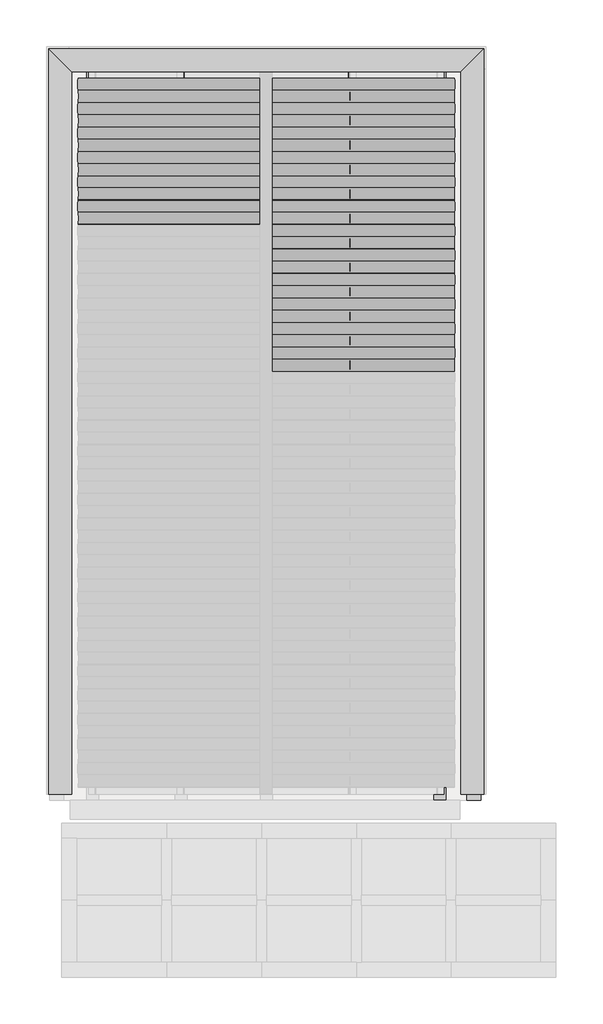
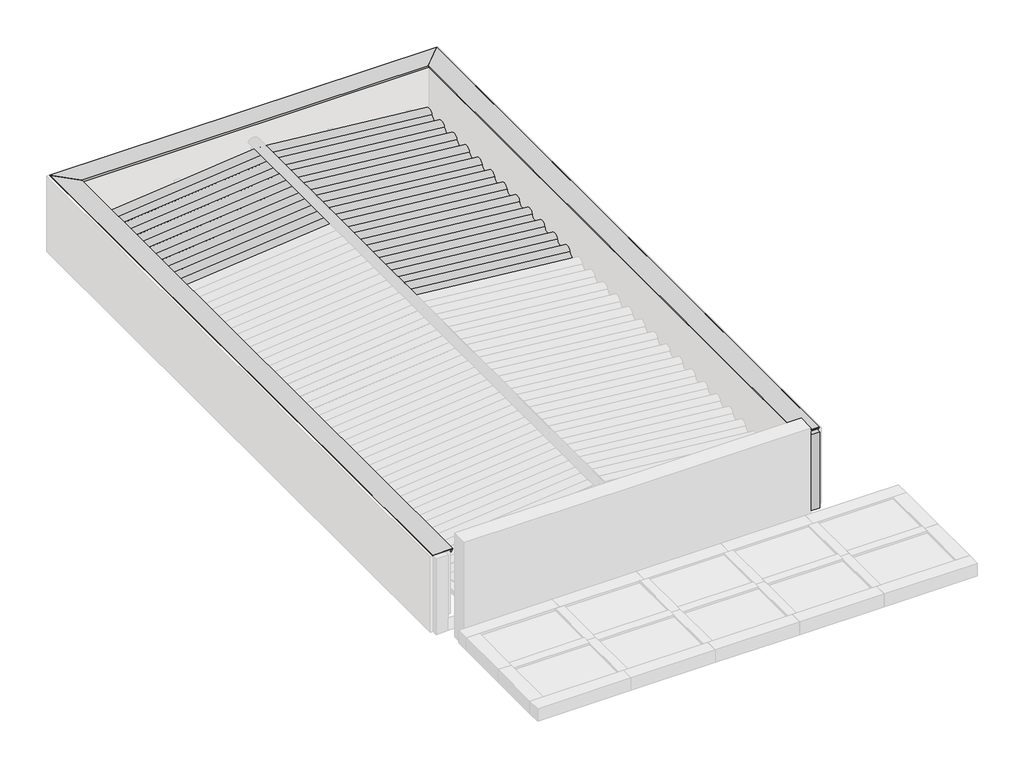
# One storey, part 3 of 3: 32 beams, 11 columns, 2 proxies.
"""IFC4 building model written with IfcOpenShell, lengths in millimetres."""

import ifcopenshell
import ifcopenshell.guid

model = None  # the IFC model being written
_history = None  # IfcOwnerHistory: only IFC2X3 demands one
_inside = {}  # id of a spatial element -> (the spatial element, [elements in it])
_under = {}  # id of a project, library or spatial element -> (it, [spatial elements below it])
_declared = {}  # id of a project -> (the project, [libraries it declares])
_typed = {}  # id of a type object -> (the type object, [elements of that type])
_made_of = {}  # id of a material, layer set ... -> (it, [elements and type objects made of it])


def new_model(schema):
    """Start an empty IFC model of exactly this schema.

    Asked for "IFC4X3", IfcOpenShell would pick the latest addendum, in which some entities
    have other attributes; the version numbers below select the first issue.
    IFC2X3 requires an IfcOwnerHistory on every rooted entity: one is made here for all.
    """
    global model, _history
    if schema == "IFC4X3":
        model = ifcopenshell.file(schema_version=(4, 3, 0, 0))
    else:
        model = ifcopenshell.file(schema=schema)
    _inside.clear()
    _under.clear()
    _declared.clear()
    _typed.clear()
    _made_of.clear()
    _history = None
    if model.schema == "IFC2X3":
        org = make("IfcOrganization", Name="unknown")
        user = make(
            "IfcPersonAndOrganization",
            ThePerson=make("IfcPerson", FamilyName="unknown"),
            TheOrganization=org,
        )
        app = make(
            "IfcApplication",
            ApplicationDeveloper=org,
            Version="unknown",
            ApplicationFullName="unknown",
            ApplicationIdentifier="unknown",
        )
        _history = make(
            "IfcOwnerHistory",
            OwningUser=user,
            OwningApplication=app,
            ChangeAction="ADDED",
            CreationDate=0,
        )
    return model


def make(cls, **values):
    """One entity of the class cls with the attributes given. An attribute that is None is left unset."""
    return model.create_entity(
        cls, **{name: value for name, value in values.items() if value is not None}
    )


def rooted(cls, **values):
    """An entity with a GlobalId (a new one), such as an element, a storey or a relation."""
    return make(cls, GlobalId=ifcopenshell.guid.new(), OwnerHistory=_history, **values)


def si_unit(unit_type, name, prefix=None):
    """IfcSIUnit, for example si_unit("LENGTHUNIT", "METRE", prefix="MILLI")."""
    return make("IfcSIUnit", UnitType=unit_type, Prefix=prefix, Name=name)


def assignment(units):
    """IfcUnitAssignment: the units of a project."""
    return None if units is None else make("IfcUnitAssignment", Units=units)


def point(xyz):
    """IfcCartesianPoint."""
    return None if xyz is None else make("IfcCartesianPoint", Coordinates=xyz)


def direction(xyz):
    """IfcDirection."""
    return None if xyz is None else make("IfcDirection", DirectionRatios=xyz)


def frame(location, z_axis=None, x_axis=None):
    """IfcAxis2Placement3D, a coordinate frame: its origin and axes. An axis left out is left unset."""
    return make(
        "IfcAxis2Placement3D",
        Location=point(location),
        Axis=direction(z_axis),
        RefDirection=direction(x_axis),
    )


def frame_2d(location, x_axis=None):
    """IfcAxis2Placement2D, a coordinate frame in the plane: its origin and x axis."""
    return make(
        "IfcAxis2Placement2D", Location=point(location), RefDirection=direction(x_axis)
    )


def origin():
    """The frame at (0, 0, 0) with its axes left unset."""
    return frame((0.0, 0.0, 0.0))


def place(relative_to, where):
    """IfcLocalPlacement: puts the frame where relative to a parent placement (None: the world)."""
    return make(
        "IfcLocalPlacement", PlacementRelTo=relative_to, RelativePlacement=where
    )


def context(
    kind, dimensions, precision=None, world=None, true_north=None, identifier=None
):
    """IfcGeometricRepresentationContext, for example the 3D "Model" context."""
    return make(
        "IfcGeometricRepresentationContext",
        ContextIdentifier=identifier,
        ContextType=kind,
        CoordinateSpaceDimension=dimensions,
        Precision=precision,
        WorldCoordinateSystem=world,
        TrueNorth=true_north,
    )


def project(units=None, contexts=None):
    """IfcProject with its units and contexts."""
    return rooted(
        "IfcProject",
        Name="project",
        RepresentationContexts=contexts,
        UnitsInContext=assignment(units),
    )


def spatial(cls, under=None, at=None, **own):
    """A site, building, storey or space (cls), placed at a placement, below another one or the project."""
    s = rooted(cls, ObjectPlacement=at, **own)
    if under is not None:
        _under.setdefault(under.id(), (under, []))[1].append(s)
    return s


def polyline(points):
    """IfcPolyline through the points."""
    return make("IfcPolyline", Points=[point(p) for p in points])


def circle_curve(where, radius):
    """IfcCircle in the frame where."""
    return make("IfcCircle", Position=where, Radius=radius)


def trimmed(basis, trim1, trim2, sense, master):
    """IfcTrimmedCurve: the piece of a basis curve between two trims."""
    return make(
        "IfcTrimmedCurve",
        BasisCurve=basis,
        Trim1=trim1,
        Trim2=trim2,
        SenseAgreement=sense,
        MasterRepresentation=master,
    )


def segment(curve, same_sense, transition):
    """IfcCompositeCurveSegment."""
    return make(
        "IfcCompositeCurveSegment",
        Transition=transition,
        SameSense=same_sense,
        ParentCurve=curve,
    )


def composite_curve(segments, self_intersect=None):
    """IfcCompositeCurve: segments joined end to end."""
    return make("IfcCompositeCurve", Segments=segments, SelfIntersect=self_intersect)


def outline(outer, holes=None, kind="AREA"):
    """IfcArbitraryClosedProfileDef: a profile drawn as a closed curve; with holes, ...WithVoids."""
    if holes is None:
        return make("IfcArbitraryClosedProfileDef", ProfileType=kind, OuterCurve=outer)
    return make(
        "IfcArbitraryProfileDefWithVoids",
        ProfileType=kind,
        OuterCurve=outer,
        InnerCurves=holes,
    )


def extrude(swept, where, along, depth):
    """IfcExtrudedAreaSolid: the profile swept, set in the frame where, extruded along a direction by depth."""
    return make(
        "IfcExtrudedAreaSolid",
        SweptArea=swept,
        Position=where,
        ExtrudedDirection=direction(along),
        Depth=depth,
    )


def faces_of(points, faces, orient=None, outer=None):
    """IfcFace entities. A face is a list of loops; a loop is a list of indices into points, from 0.

    orient and outer hold one flag for each loop. By default every Orientation is true, the
    first loop of a face is its IfcFaceOuterBound and the others are IfcFaceBound.
    """
    made = []
    for i, loops in enumerate(faces):
        bounds = []
        for j, loop in enumerate(loops):
            is_outer = j == 0 if outer is None else outer[i][j]
            bounds.append(
                make(
                    "IfcFaceOuterBound" if is_outer else "IfcFaceBound",
                    Bound=make("IfcPolyLoop", Polygon=[points[k] for k in loop]),
                    Orientation=True if orient is None else orient[i][j],
                )
            )
        made.append(make("IfcFace", Bounds=bounds))
    return made


def faceted_brep(points, faces, orient=None, outer=None, voids=None):
    """IfcFacetedBrep: a solid bounded by flat faces; with voids (closed shells), ...WithVoids."""
    shared = [point(p) for p in points]
    hull = make("IfcClosedShell", CfsFaces=faces_of(shared, faces, orient, outer))
    if voids is None:
        return make("IfcFacetedBrep", Outer=hull)
    return make(
        "IfcFacetedBrepWithVoids",
        Outer=hull,
        Voids=[
            make(cls, CfsFaces=faces_of(shared, fs, o, b)) for cls, fs, o, b in voids
        ],
    )


def shape(context_of_items, identifier, shape_type, items):
    """IfcShapeRepresentation: the items that make up one representation, for example the "Body"."""
    return make(
        "IfcShapeRepresentation",
        ContextOfItems=context_of_items,
        RepresentationIdentifier=identifier,
        RepresentationType=shape_type,
        Items=items,
    )


def source(mapping_origin, context_of_items, identifier, shape_type, items):
    """IfcRepresentationMap: a shape defined once, which mapped items show again and again."""
    return make(
        "IfcRepresentationMap",
        MappingOrigin=mapping_origin,
        MappedRepresentation=shape(context_of_items, identifier, shape_type, items),
    )


def transform(
    local_origin,
    x_axis=None,
    y_axis=None,
    z_axis=None,
    scale=None,
    scale2=None,
    scale3=None,
    uniform=True,
):
    """IfcCartesianTransformationOperator3D, or its non-uniform kind. x_axis, y_axis, z_axis: its Axis1, 2, 3."""
    if uniform:
        return make(
            "IfcCartesianTransformationOperator3D",
            Axis1=direction(x_axis),
            Axis2=direction(y_axis),
            LocalOrigin=point(local_origin),
            Scale=scale,
            Axis3=direction(z_axis),
        )
    return make(
        "IfcCartesianTransformationOperator3DnonUniform",
        Axis1=direction(x_axis),
        Axis2=direction(y_axis),
        LocalOrigin=point(local_origin),
        Scale=scale,
        Axis3=direction(z_axis),
        Scale2=scale2,
        Scale3=scale3,
    )


def mapped(mapping_source, mapping_target):
    """IfcMappedItem: shows the shape of a source again, moved by a transform."""
    return make(
        "IfcMappedItem", MappingSource=mapping_source, MappingTarget=mapping_target
    )


def made_of(thing, what):
    """Note that an element or type object is made of a material, layer set ...; save() writes the relation."""
    if what is not None:
        _made_of.setdefault(what.id(), (what, []))[1].append(thing)
    return thing


def element(
    cls,
    number,
    at=None,
    inside=None,
    cuts=None,
    type_object=None,
    material=None,
    context=None,
    identifier="Body",
    shape_type=None,
    held_by="IfcProductDefinitionShape",
    body=None,
    shapes=None,
    **own,
):
    """One element of the class cls, such as IfcWall. Its Tag is "e" and its number.

    at: its placement. inside: the storey or other place that contains it. cuts: it is an
    opening in that element (IfcRelVoidsElement). A single representation is given by context,
    identifier, shape_type and body (its items); several are given by shapes. held_by: the class
    of the entity that holds the representations. save() writes the other relations.
    """
    e = rooted(cls, Tag="e%d" % number, ObjectPlacement=at, **own)
    if body is not None:
        shapes = [shape(context, identifier, shape_type, body)]
    if shapes is not None:
        e.Representation = make(held_by, Representations=shapes)
    if inside is not None:
        _inside.setdefault(inside.id(), (inside, []))[1].append(e)
    if cuts is not None:
        rooted(
            "IfcRelVoidsElement", RelatingBuildingElement=cuts, RelatedOpeningElement=e
        )
    if type_object is not None:
        _typed.setdefault(type_object.id(), (type_object, []))[1].append(e)
    return made_of(e, material)


def aggregate(whole, parts):
    """IfcRelAggregates: a whole, such as a stair, and the parts it consists of."""
    return rooted("IfcRelAggregates", RelatingObject=whole, RelatedObjects=parts)


def save(model, path):
    """Write the relations noted so far, then the file.

    IfcRelAggregates (storeys below a building ...), IfcRelContainedInSpatialStructure (elements
    in a storey), IfcRelDefinesByType, IfcRelAssociatesMaterial and IfcRelDeclares: one each for
    every whole, place, type object, material and project.
    """
    for whole, parts in _under.values():
        aggregate(whole, parts)
    for where, things in _inside.values():
        rooted(
            "IfcRelContainedInSpatialStructure",
            RelatedElements=things,
            RelatingStructure=where,
        )
    for kind, things in _typed.values():
        rooted("IfcRelDefinesByType", RelatedObjects=things, RelatingType=kind)
    for what, things in _made_of.values():
        rooted("IfcRelAssociatesMaterial", RelatedObjects=things, RelatingMaterial=what)
    for by, libraries in _declared.values():
        rooted("IfcRelDeclares", RelatingContext=by, RelatedDefinitions=libraries)
    model.write(path)


def column_1cffec27(model_context):
    return source(origin(), model_context, "Body", "SweptSolid", [
        extrude(outline(polyline([(30.0, 80.0), (30.0, -80.0), (-30.0, -80.0), (-30.0, 80.0), (30.0, 80.0)])), frame((0.0, 0.0, 3110.0), z_axis=(0.0, 0.0, 1.0), x_axis=(1.0, 0.0, 0.0)), (0.0, 0.0, 1.0), 238.0),
    ])


def column_35730ad5(model_context):
    return source(origin(), model_context, "Body", "SweptSolid", [
        extrude(outline(polyline([(30.0, 80.0), (30.0, -80.0), (-30.0, -80.0), (-30.0, 80.0), (30.0, 80.0)])), frame((0.0, 0.0, 3110.0), z_axis=(0.0, 0.0, 1.0), x_axis=(1.0, 0.0, 0.0)), (0.0, 0.0, 1.0), 197.9),
    ])


def column_00c463e4(model_context):
    return source(origin(), model_context, "Body", "SweptSolid", [
        extrude(outline(polyline([(30.0, 80.0), (30.0, -80.0), (-30.0, -80.0), (-30.0, 80.0), (30.0, 80.0)])), frame((0.0, 0.0, 3110.0), z_axis=(0.0, 0.0, 1.0), x_axis=(1.0, 0.0, 0.0)), (0.0, 0.0, 1.0), 109.8),
    ])


model = new_model("IFC4")

# Units and contexts
model_context = context("Model", 3, world=origin())
ifc_project = project(units=[si_unit("LENGTHUNIT", "METRE", prefix="MILLI")], contexts=[model_context])

# Site, building, storey
site = spatial("IfcSite", under=ifc_project)
building = spatial("IfcBuilding", under=site)
storey = spatial("IfcBuildingStorey", under=building, Name="COB. GARAGEM", Elevation=3050.0)

# Beams
placement = place(None, origin())
element("IfcBeam", 1, ObjectType="Madeira de lei : Berço 6x12cm", at=placement, inside=storey, context=model_context, shape_type="SweptSolid", body=[
    extrude(outline(polyline([(-9620.281307, 6423.9300153), (-9500.281307, 6423.9300153), (-9500.281307, 4423.9300153), (-9620.281307, 4423.9300153), (-9620.281307, 6423.9300153)])), frame((0.0, 0.0, 3050.0), z_axis=(0.0, 0.0, 1.0), x_axis=(1.0, 0.0, 0.0)), (0.0, 0.0, 1.0), 60.0),
])
element("IfcBeam", 2, ObjectType="Madeira de lei : Berço 6x12cm", at=placement, inside=storey, context=model_context, shape_type="SweptSolid", body=[
    extrude(outline(polyline([(-9620.281307, 7083.9300153), (-9500.281307, 7083.9300153), (-9500.281307, 6423.9300153), (-9620.281307, 6423.9300153), (-9620.281307, 7083.9300153)])), frame((0.0, 0.0, 3050.0), z_axis=(0.0, 0.0, 1.0), x_axis=(1.0, 0.0, 0.0)), (0.0, 0.0, 1.0), 60.0),
])
element("IfcBeam", 3, ObjectType="Madeira de lei : Berço 6x12cm", at=placement, inside=storey, context=model_context, shape_type="SweptSolid", body=[
    extrude(outline(polyline([(-8767.0824227, 6423.9300153), (-8647.0824227, 6423.9300153), (-8647.0824227, 4423.9300153), (-8767.0824227, 4423.9300153), (-8767.0824227, 6423.9300153)])), frame((0.0, 0.0, 3050.0), z_axis=(0.0, 0.0, 1.0), x_axis=(1.0, 0.0, 0.0)), (0.0, 0.0, 1.0), 60.0),
])
element("IfcBeam", 4, ObjectType="Madeira de lei : Berço 6x12cm", at=placement, inside=storey, context=model_context, shape_type="SweptSolid", body=[
    extrude(outline(polyline([(-8767.0824227, 7083.9300153), (-8647.0824227, 7083.9300153), (-8647.0824227, 6423.9300153), (-8767.0824227, 6423.9300153), (-8767.0824227, 7083.9300153)])), frame((0.0, 0.0, 3050.0), z_axis=(0.0, 0.0, 1.0), x_axis=(1.0, 0.0, 0.0)), (0.0, 0.0, 1.0), 60.0),
])
element("IfcBeam", 5, ObjectType="Madeira de lei : Berço 6x12cm", at=placement, inside=storey, context=model_context, shape_type="SweptSolid", body=[
    extrude(outline(polyline([(-7884.0324227, 4423.9300153), (-7764.0324227, 4423.9300153), (-7764.0324227, 2423.9300153), (-7884.0324227, 2423.9300153), (-7884.0324227, 4423.9300153)])), frame((0.0, 0.0, 3050.0), z_axis=(0.0, 0.0, 1.0), x_axis=(1.0, 0.0, 0.0)), (0.0, 0.0, 1.0), 60.0),
])
element("IfcBeam", 6, ObjectType="Madeira de lei : Berço 6x12cm", at=placement, inside=storey, context=model_context, shape_type="SweptSolid", body=[
    extrude(outline(polyline([(-7884.0324227, 6423.9300153), (-7764.0324227, 6423.9300153), (-7764.0324227, 4423.9300153), (-7884.0324227, 4423.9300153), (-7884.0324227, 6423.9300153)])), frame((0.0, 0.0, 3050.0), z_axis=(0.0, 0.0, 1.0), x_axis=(1.0, 0.0, 0.0)), (0.0, 0.0, 1.0), 60.0),
])
element("IfcBeam", 7, ObjectType="Madeira de lei : Berço 6x12cm", at=placement, inside=storey, context=model_context, shape_type="SweptSolid", body=[
    extrude(outline(polyline([(-7884.0324227, 2423.9300153), (-7764.0324227, 2423.9300153), (-7764.0324227, 423.9300153), (-7884.0324227, 423.9300153), (-7884.0324227, 2423.9300153)])), frame((0.0, 0.0, 3050.0), z_axis=(0.0, 0.0, 1.0), x_axis=(1.0, 0.0, 0.0)), (0.0, 0.0, 1.0), 60.0),
])
element("IfcBeam", 8, ObjectType="Madeira de lei : Berço 6x12cm", at=placement, inside=storey, context=model_context, shape_type="SweptSolid", body=[
    extrude(outline(polyline([(-7884.0324227, 7083.9300153), (-7764.0324227, 7083.9300153), (-7764.0324227, 6423.9300153), (-7884.0324227, 6423.9300153), (-7884.0324227, 7083.9300153)])), frame((0.0, 0.0, 3050.0), z_axis=(0.0, 0.0, 1.0), x_axis=(1.0, 0.0, 0.0)), (0.0, 0.0, 1.0), 60.0),
])
element("IfcBeam", 9, ObjectType="Madeira de lei : Berço 6x12cm", at=placement, inside=storey, context=model_context, shape_type="SweptSolid", body=[
    extrude(outline(polyline([(-7884.0324227, 423.9300153), (-7764.0324227, 423.9300153), (-7764.0324227, -236.0699847), (-7884.0324227, -236.0699847), (-7884.0324227, 423.9300153)])), frame((0.0, 0.0, 3050.0), z_axis=(0.0, 0.0, 1.0), x_axis=(1.0, 0.0, 0.0)), (0.0, 0.0, 1.0), 60.0),
])
element("IfcBeam", 10, ObjectType="Madeira de lei : Berço 6x12cm", at=placement, inside=storey, context=model_context, shape_type="SweptSolid", body=[
    extrude(outline(polyline([(-10473.4801913, 6423.9300153), (-10353.4801913, 6423.9300153), (-10353.4801913, 4423.9300153), (-10473.4801913, 4423.9300153), (-10473.4801913, 6423.9300153)])), frame((0.0, 0.0, 3050.0), z_axis=(0.0, 0.0, 1.0), x_axis=(1.0, 0.0, 0.0)), (0.0, 0.0, 1.0), 60.0),
])
element("IfcBeam", 11, ObjectType="Madeira de lei : Berço 6x12cm", at=placement, inside=storey, context=model_context, shape_type="SweptSolid", body=[
    extrude(outline(polyline([(-10473.4801913, 7083.9300153), (-10353.4801913, 7083.9300153), (-10353.4801913, 6423.9300153), (-10473.4801913, 6423.9300153), (-10473.4801913, 7083.9300153)])), frame((0.0, 0.0, 3050.0), z_axis=(0.0, 0.0, 1.0), x_axis=(1.0, 0.0, 0.0)), (0.0, 0.0, 1.0), 60.0),
])
element("IfcBeam", 12, ObjectType="Madeira de lei : Berço 6x12cm", at=placement, inside=storey, context=model_context, shape_type="SweptSolid", body=[
    extrude(outline(polyline([(-11356.5301913, 7083.9300153), (-11236.5301913, 7083.9300153), (-11236.5301913, 6423.9300153), (-11356.5301913, 6423.9300153), (-11356.5301913, 7083.9300153)])), frame((0.0, 0.0, 3050.0), z_axis=(0.0, 0.0, 1.0), x_axis=(1.0, 0.0, 0.0)), (0.0, 0.0, 1.0), 60.0),
])
element("IfcBeam", 13, ObjectType="TQS - Viga retangular : 14.0 x 90.0", at=placement, inside=storey, context=model_context, shape_type="Brep", body=[
    faceted_brep([(-7712.281307, 7134.4300153, 3800.0), (-7712.281307, 7274.4300153, 3800.0), (-11430.281307, 7274.4300153, 3800.0), (-11430.281307, 7134.4300153, 3800.0), (-7712.281307, 7134.4300153, 2900.0), (-7712.281307, 7134.4300153, 3050.0), (-11430.281307, 7134.4300153, 3050.0), (-11430.281307, 7134.4300153, 2900.0), (-7712.281307, 7274.4300153, 2900.0), (-11430.281307, 7274.4300153, 2900.0)], [[[0, 1, 2, 3]], [[4, 5, 0, 3, 6, 7]], [[8, 4, 7, 9]], [[1, 8, 9, 2]], [[2, 9, 7, 6, 3]], [[1, 0, 5, 4, 8]]]),
])
element("IfcBeam", 14, ObjectType="TQS - Viga retangular : 14.0 x 90.0", at=placement, inside=storey, context=model_context, shape_type="Brep", body=[
    faceted_brep([(-7412.281307, 7084.4300153, 3800.0), (-7552.281307, 7084.4300153, 3800.0), (-7552.281307, -234.5699847, 3800.0), (-7412.281307, -234.5699847, 3800.0), (-7412.281307, 7084.4300153, 2900.0), (-7412.281307, -234.5699847, 2900.0), (-7552.281307, 7084.4300153, 2900.0), (-7552.281307, -234.5699847, 2900.0), (-7552.281307, 7084.4300153, 3050.0), (-7552.281307, -234.5699847, 3050.0)], [[[0, 1, 2, 3]], [[4, 0, 3, 5]], [[6, 4, 5, 7]], [[1, 8, 6, 7, 9, 2]], [[2, 9, 7, 5, 3]], [[1, 0, 4, 6, 8]]]),
])
element("IfcBeam", 15, ObjectType="Telha Ondulada : Fibrocimento", at=placement, inside=storey, context=model_context, shape_type="SweptSolid", body=[
    extrude(outline(composite_curve([segment(trimmed(circle_curve(frame_2d((-58.7002979, -53.2060538)), 66.7939461), [point((-29.350149, 6.7939462))], [point((-29.350149, -113.2060538))], False, "CARTESIAN"), True, "CONTINUOUS"), segment(polyline([(-29.350149, -113.2060538), (-31.5472155, -108.7146288)]), True, "CONTINUOUS"), segment(trimmed(circle_curve(frame_2d((-58.7002979, -53.2060538)), 61.7939461), [point((-31.5472155, -108.7146288))], [point((-31.5472155, 2.3025211))], True, "CARTESIAN"), True, "CONTINUOUS"), segment(trimmed(circle_curve(frame_2d((0.0, 66.7939462)), 71.7939461), [point((-31.5472155, 2.3025211))], [point((-31.5472155, 131.2853712))], False, "CARTESIAN"), True, "CONTINUOUS"), segment(polyline([(-31.5472155, 131.2853712), (-29.350149, 126.7939462)]), True, "CONTINUOUS"), segment(trimmed(circle_curve(frame_2d((0.0, 66.7939462)), 66.7939461), [point((-29.350149, 126.7939462))], [point((-29.350149, 6.7939462))], True, "CARTESIAN"), True, "CONTINUOUS")], self_intersect=False)), frame((-11446.918865, 5652.326948, 3394.3067746), z_axis=(0.9950371902099892, 0.0, 0.09950371902099954), x_axis=(-0.09950371902099954, 0.0, 0.9950371902099892)), (0.0, 0.0, 1.0), 1886.8678854),
])
element("IfcBeam", 16, ObjectType="Telha Ondulada : Fibrocimento", at=placement, inside=storey, context=model_context, shape_type="SweptSolid", body=[
    extrude(outline(composite_curve([segment(trimmed(circle_curve(frame_2d((-58.7002979, -53.2060538)), 66.7939461), [point((-29.350149, 6.7939462))], [point((-29.350149, -113.2060538))], False, "CARTESIAN"), True, "CONTINUOUS"), segment(polyline([(-29.350149, -113.2060538), (-31.5472155, -108.7146288)]), True, "CONTINUOUS"), segment(trimmed(circle_curve(frame_2d((-58.7002979, -53.2060538)), 61.7939461), [point((-31.5472155, -108.7146288))], [point((-31.5472155, 2.3025211))], True, "CARTESIAN"), True, "CONTINUOUS"), segment(trimmed(circle_curve(frame_2d((0.0, 66.7939462)), 71.7939461), [point((-31.5472155, 2.3025211))], [point((-31.5472155, 131.2853712))], False, "CARTESIAN"), True, "CONTINUOUS"), segment(polyline([(-31.5472155, 131.2853712), (-29.350149, 126.7939462)]), True, "CONTINUOUS"), segment(trimmed(circle_curve(frame_2d((0.0, 66.7939462)), 66.7939461), [point((-29.350149, 126.7939462))], [point((-29.350149, 6.7939462))], True, "CARTESIAN"), True, "CONTINUOUS")], self_intersect=False)), frame((-11446.918865, 5896.826948, 3394.3067746), z_axis=(0.9950371902099892, 0.0, 0.09950371902099932), x_axis=(-0.09950371902099932, 0.0, 0.9950371902099892)), (0.0, 0.0, 1.0), 1886.8678854),
])
element("IfcBeam", 17, ObjectType="Telha Ondulada : Fibrocimento", at=placement, inside=storey, context=model_context, shape_type="SweptSolid", body=[
    extrude(outline(composite_curve([segment(trimmed(circle_curve(frame_2d((-58.7002979, -53.2060538)), 66.7939461), [point((-29.350149, 6.7939462))], [point((-29.350149, -113.2060538))], False, "CARTESIAN"), True, "CONTINUOUS"), segment(polyline([(-29.350149, -113.2060538), (-31.5472155, -108.7146288)]), True, "CONTINUOUS"), segment(trimmed(circle_curve(frame_2d((-58.7002979, -53.2060538)), 61.7939461), [point((-31.5472155, -108.7146288))], [point((-31.5472155, 2.3025211))], True, "CARTESIAN"), True, "CONTINUOUS"), segment(trimmed(circle_curve(frame_2d((0.0, 66.7939462)), 71.7939461), [point((-31.5472155, 2.3025211))], [point((-31.5472155, 131.2853712))], False, "CARTESIAN"), True, "CONTINUOUS"), segment(polyline([(-31.5472155, 131.2853712), (-29.350149, 126.7939462)]), True, "CONTINUOUS"), segment(trimmed(circle_curve(frame_2d((0.0, 66.7939462)), 66.7939461), [point((-29.350149, 126.7939462))], [point((-29.350149, 6.7939462))], True, "CARTESIAN"), True, "CONTINUOUS")], self_intersect=False)), frame((-11446.918865, 6141.326948, 3394.3067746), z_axis=(0.9950371902099892, 0.0, 0.09950371902099943), x_axis=(-0.09950371902099943, 0.0, 0.9950371902099892)), (0.0, 0.0, 1.0), 1886.8678854),
])
element("IfcBeam", 18, ObjectType="Telha Ondulada : Fibrocimento", at=placement, inside=storey, context=model_context, shape_type="SweptSolid", body=[
    extrude(outline(composite_curve([segment(trimmed(circle_curve(frame_2d((-58.7002979, -53.2060538)), 66.7939461), [point((-29.350149, 6.7939462))], [point((-29.350149, -113.2060538))], False, "CARTESIAN"), True, "CONTINUOUS"), segment(polyline([(-29.350149, -113.2060538), (-31.5472155, -108.7146288)]), True, "CONTINUOUS"), segment(trimmed(circle_curve(frame_2d((-58.7002979, -53.2060538)), 61.7939461), [point((-31.5472155, -108.7146288))], [point((-31.5472155, 2.3025211))], True, "CARTESIAN"), True, "CONTINUOUS"), segment(trimmed(circle_curve(frame_2d((0.0, 66.7939462)), 71.7939461), [point((-31.5472155, 2.3025211))], [point((-31.5472155, 131.2853712))], False, "CARTESIAN"), True, "CONTINUOUS"), segment(polyline([(-31.5472155, 131.2853712), (-29.350149, 126.7939462)]), True, "CONTINUOUS"), segment(trimmed(circle_curve(frame_2d((0.0, 66.7939462)), 66.7939461), [point((-29.350149, 126.7939462))], [point((-29.350149, 6.7939462))], True, "CARTESIAN"), True, "CONTINUOUS")], self_intersect=False)), frame((-11446.918865, 6385.826948, 3394.3067746), z_axis=(0.9950371902099892, 0.0, 0.09950371902099919), x_axis=(-0.09950371902099919, 0.0, 0.9950371902099892)), (0.0, 0.0, 1.0), 1886.8678854),
])
element("IfcBeam", 19, ObjectType="Telha Ondulada : Fibrocimento", at=placement, inside=storey, context=model_context, shape_type="SweptSolid", body=[
    extrude(outline(composite_curve([segment(trimmed(circle_curve(frame_2d((-58.7002979, -53.2060538)), 66.7939461), [point((-29.350149, 6.7939462))], [point((-29.350149, -113.2060538))], False, "CARTESIAN"), True, "CONTINUOUS"), segment(polyline([(-29.350149, -113.2060538), (-31.5472155, -108.7146288)]), True, "CONTINUOUS"), segment(trimmed(circle_curve(frame_2d((-58.7002979, -53.2060538)), 61.7939461), [point((-31.5472155, -108.7146288))], [point((-31.5472155, 2.3025211))], True, "CARTESIAN"), True, "CONTINUOUS"), segment(trimmed(circle_curve(frame_2d((0.0, 66.7939462)), 71.7939461), [point((-31.5472155, 2.3025211))], [point((-31.5472155, 131.2853712))], False, "CARTESIAN"), True, "CONTINUOUS"), segment(polyline([(-31.5472155, 131.2853712), (-29.350149, 126.7939462)]), True, "CONTINUOUS"), segment(trimmed(circle_curve(frame_2d((0.0, 66.7939462)), 66.7939461), [point((-29.350149, 126.7939462))], [point((-29.350149, 6.7939462))], True, "CARTESIAN"), True, "CONTINUOUS")], self_intersect=False)), frame((-11446.918865, 6630.326948, 3394.3067746), z_axis=(0.9950371902099892, 0.0, 0.09950371902099925), x_axis=(-0.09950371902099925, 0.0, 0.9950371902099892)), (0.0, 0.0, 1.0), 1886.8678854),
])
element("IfcBeam", 20, ObjectType="Telha Ondulada : Fibrocimento", at=placement, inside=storey, context=model_context, shape_type="SweptSolid", body=[
    extrude(outline(composite_curve([segment(trimmed(circle_curve(frame_2d((-58.7002979, -53.2060538)), 66.7939461), [point((-29.350149, 6.7939462))], [point((-29.350149, -113.2060538))], False, "CARTESIAN"), True, "CONTINUOUS"), segment(polyline([(-29.350149, -113.2060538), (-31.5472155, -108.7146288)]), True, "CONTINUOUS"), segment(trimmed(circle_curve(frame_2d((-58.7002979, -53.2060538)), 61.7939461), [point((-31.5472155, -108.7146288))], [point((-31.5472155, 2.3025211))], True, "CARTESIAN"), True, "CONTINUOUS"), segment(trimmed(circle_curve(frame_2d((0.0, 66.7939462)), 71.7939461), [point((-31.5472155, 2.3025211))], [point((-31.5472155, 131.2853712))], False, "CARTESIAN"), True, "CONTINUOUS"), segment(polyline([(-31.5472155, 131.2853712), (-29.350149, 126.7939462)]), True, "CONTINUOUS"), segment(trimmed(circle_curve(frame_2d((0.0, 66.7939462)), 66.7939461), [point((-29.350149, 126.7939462))], [point((-29.350149, 6.7939462))], True, "CARTESIAN"), True, "CONTINUOUS")], self_intersect=False)), frame((-11446.918865, 6874.826948, 3394.3067746), z_axis=(0.9950371902099892, 0.0, 0.09950371902099937), x_axis=(-0.09950371902099937, 0.0, 0.9950371902099892)), (0.0, 0.0, 1.0), 1886.8678854),
])
element("IfcBeam", 21, ObjectType="Telha Ondulada : Fibrocimento", at=placement, inside=storey, context=model_context, shape_type="SweptSolid", body=[
    extrude(outline(composite_curve([segment(trimmed(circle_curve(frame_2d((0.0, 66.7939462)), 66.7939461), [point((29.350149, 6.7939462))], [point((29.350149, 126.7939462))], True, "CARTESIAN"), True, "CONTINUOUS"), segment(polyline([(29.350149, 126.7939462), (31.5472155, 131.2853712)]), True, "CONTINUOUS"), segment(trimmed(circle_curve(frame_2d((0.0, 66.7939462)), 71.7939461), [point((31.5472155, 131.2853712))], [point((31.5472155, 2.3025211))], False, "CARTESIAN"), True, "CONTINUOUS"), segment(trimmed(circle_curve(frame_2d((58.7002979, -53.2060538)), 61.7939461), [point((31.5472155, 2.3025211))], [point((31.5472155, -108.7146288))], True, "CARTESIAN"), True, "CONTINUOUS"), segment(polyline([(31.5472155, -108.7146288), (29.350149, -113.2060538)]), True, "CONTINUOUS"), segment(trimmed(circle_curve(frame_2d((58.7002979, -53.2060538)), 66.7939461), [point((29.350149, -113.2060538))], [point((29.350149, 6.7939462))], False, "CARTESIAN"), True, "CONTINUOUS")], self_intersect=False)), frame((-7673.6437489, 4185.326948, 3394.3067746), z_axis=(-0.9950371902099892, 0.0, 0.09950371902099965), x_axis=(-0.09950371902099965, 0.0, -0.9950371902099892)), (0.0, 0.0, 1.0), 1886.8678854),
])
element("IfcBeam", 22, ObjectType="Telha Ondulada : Fibrocimento", at=placement, inside=storey, context=model_context, shape_type="SweptSolid", body=[
    extrude(outline(composite_curve([segment(trimmed(circle_curve(frame_2d((0.0, 66.7939462)), 66.7939461), [point((29.350149, 6.7939462))], [point((29.350149, 126.7939462))], True, "CARTESIAN"), True, "CONTINUOUS"), segment(polyline([(29.350149, 126.7939462), (31.5472155, 131.2853712)]), True, "CONTINUOUS"), segment(trimmed(circle_curve(frame_2d((0.0, 66.7939462)), 71.7939461), [point((31.5472155, 131.2853712))], [point((31.5472155, 2.3025211))], False, "CARTESIAN"), True, "CONTINUOUS"), segment(trimmed(circle_curve(frame_2d((58.7002979, -53.2060538)), 61.7939461), [point((31.5472155, 2.3025211))], [point((31.5472155, -108.7146288))], True, "CARTESIAN"), True, "CONTINUOUS"), segment(polyline([(31.5472155, -108.7146288), (29.350149, -113.2060538)]), True, "CONTINUOUS"), segment(trimmed(circle_curve(frame_2d((58.7002979, -53.2060538)), 66.7939461), [point((29.350149, -113.2060538))], [point((29.350149, 6.7939462))], False, "CARTESIAN"), True, "CONTINUOUS")], self_intersect=False)), frame((-7673.6437489, 4429.826948, 3394.3067746), z_axis=(-0.9950371902099892, 0.0, 0.09950371902099965), x_axis=(-0.09950371902099965, 0.0, -0.9950371902099892)), (0.0, 0.0, 1.0), 1886.8678854),
])
element("IfcBeam", 23, ObjectType="Telha Ondulada : Fibrocimento", at=placement, inside=storey, context=model_context, shape_type="SweptSolid", body=[
    extrude(outline(composite_curve([segment(trimmed(circle_curve(frame_2d((0.0, 66.7939462)), 66.7939461), [point((29.350149, 6.7939462))], [point((29.350149, 126.7939462))], True, "CARTESIAN"), True, "CONTINUOUS"), segment(polyline([(29.350149, 126.7939462), (31.5472155, 131.2853712)]), True, "CONTINUOUS"), segment(trimmed(circle_curve(frame_2d((0.0, 66.7939462)), 71.7939461), [point((31.5472155, 131.2853712))], [point((31.5472155, 2.3025211))], False, "CARTESIAN"), True, "CONTINUOUS"), segment(trimmed(circle_curve(frame_2d((58.7002979, -53.2060538)), 61.7939461), [point((31.5472155, 2.3025211))], [point((31.5472155, -108.7146288))], True, "CARTESIAN"), True, "CONTINUOUS"), segment(polyline([(31.5472155, -108.7146288), (29.350149, -113.2060538)]), True, "CONTINUOUS"), segment(trimmed(circle_curve(frame_2d((58.7002979, -53.2060538)), 66.7939461), [point((29.350149, -113.2060538))], [point((29.350149, 6.7939462))], False, "CARTESIAN"), True, "CONTINUOUS")], self_intersect=False)), frame((-7673.6437489, 4674.326948, 3394.3067746), z_axis=(-0.9950371902099892, 0.0, 0.09950371902099965), x_axis=(-0.09950371902099965, 0.0, -0.9950371902099892)), (0.0, 0.0, 1.0), 1886.8678854),
])
element("IfcBeam", 24, ObjectType="Telha Ondulada : Fibrocimento", at=placement, inside=storey, context=model_context, shape_type="SweptSolid", body=[
    extrude(outline(composite_curve([segment(trimmed(circle_curve(frame_2d((0.0, 66.7939462)), 66.7939461), [point((29.350149, 6.7939462))], [point((29.350149, 126.7939462))], True, "CARTESIAN"), True, "CONTINUOUS"), segment(polyline([(29.350149, 126.7939462), (31.5472155, 131.2853712)]), True, "CONTINUOUS"), segment(trimmed(circle_curve(frame_2d((0.0, 66.7939462)), 71.7939461), [point((31.5472155, 131.2853712))], [point((31.5472155, 2.3025211))], False, "CARTESIAN"), True, "CONTINUOUS"), segment(trimmed(circle_curve(frame_2d((58.7002979, -53.2060538)), 61.7939461), [point((31.5472155, 2.3025211))], [point((31.5472155, -108.7146288))], True, "CARTESIAN"), True, "CONTINUOUS"), segment(polyline([(31.5472155, -108.7146288), (29.350149, -113.2060538)]), True, "CONTINUOUS"), segment(trimmed(circle_curve(frame_2d((58.7002979, -53.2060538)), 66.7939461), [point((29.350149, -113.2060538))], [point((29.350149, 6.7939462))], False, "CARTESIAN"), True, "CONTINUOUS")], self_intersect=False)), frame((-7673.6437489, 4918.826948, 3394.3067746), z_axis=(-0.9950371902099892, 0.0, 0.09950371902099965), x_axis=(-0.09950371902099965, 0.0, -0.9950371902099892)), (0.0, 0.0, 1.0), 1886.8678854),
])
element("IfcBeam", 25, ObjectType="Telha Ondulada : Fibrocimento", at=placement, inside=storey, context=model_context, shape_type="SweptSolid", body=[
    extrude(outline(composite_curve([segment(trimmed(circle_curve(frame_2d((0.0, 66.7939462)), 66.7939461), [point((29.350149, 6.7939462))], [point((29.350149, 126.7939462))], True, "CARTESIAN"), True, "CONTINUOUS"), segment(polyline([(29.350149, 126.7939462), (31.5472155, 131.2853712)]), True, "CONTINUOUS"), segment(trimmed(circle_curve(frame_2d((0.0, 66.7939462)), 71.7939461), [point((31.5472155, 131.2853712))], [point((31.5472155, 2.3025211))], False, "CARTESIAN"), True, "CONTINUOUS"), segment(trimmed(circle_curve(frame_2d((58.7002979, -53.2060538)), 61.7939461), [point((31.5472155, 2.3025211))], [point((31.5472155, -108.7146288))], True, "CARTESIAN"), True, "CONTINUOUS"), segment(polyline([(31.5472155, -108.7146288), (29.350149, -113.2060538)]), True, "CONTINUOUS"), segment(trimmed(circle_curve(frame_2d((58.7002979, -53.2060538)), 66.7939461), [point((29.350149, -113.2060538))], [point((29.350149, 6.7939462))], False, "CARTESIAN"), True, "CONTINUOUS")], self_intersect=False)), frame((-7673.6437489, 5163.326948, 3394.3067746), z_axis=(-0.9950371902099892, 0.0, 0.09950371902099965), x_axis=(-0.09950371902099965, 0.0, -0.9950371902099892)), (0.0, 0.0, 1.0), 1886.8678854),
])
element("IfcBeam", 26, ObjectType="Telha Ondulada : Fibrocimento", at=placement, inside=storey, context=model_context, shape_type="SweptSolid", body=[
    extrude(outline(composite_curve([segment(trimmed(circle_curve(frame_2d((0.0, 66.7939462)), 66.7939461), [point((29.350149, 6.7939462))], [point((29.350149, 126.7939462))], True, "CARTESIAN"), True, "CONTINUOUS"), segment(polyline([(29.350149, 126.7939462), (31.5472155, 131.2853712)]), True, "CONTINUOUS"), segment(trimmed(circle_curve(frame_2d((0.0, 66.7939462)), 71.7939461), [point((31.5472155, 131.2853712))], [point((31.5472155, 2.3025211))], False, "CARTESIAN"), True, "CONTINUOUS"), segment(trimmed(circle_curve(frame_2d((58.7002979, -53.2060538)), 61.7939461), [point((31.5472155, 2.3025211))], [point((31.5472155, -108.7146288))], True, "CARTESIAN"), True, "CONTINUOUS"), segment(polyline([(31.5472155, -108.7146288), (29.350149, -113.2060538)]), True, "CONTINUOUS"), segment(trimmed(circle_curve(frame_2d((58.7002979, -53.2060538)), 66.7939461), [point((29.350149, -113.2060538))], [point((29.350149, 6.7939462))], False, "CARTESIAN"), True, "CONTINUOUS")], self_intersect=False)), frame((-7673.6437489, 5407.826948, 3394.3067746), z_axis=(-0.9950371902099892, 0.0, 0.09950371902099965), x_axis=(-0.09950371902099965, 0.0, -0.9950371902099892)), (0.0, 0.0, 1.0), 1886.8678854),
])
element("IfcBeam", 27, ObjectType="Telha Ondulada : Fibrocimento", at=placement, inside=storey, context=model_context, shape_type="SweptSolid", body=[
    extrude(outline(composite_curve([segment(trimmed(circle_curve(frame_2d((0.0, 66.7939462)), 66.7939461), [point((29.350149, 6.7939462))], [point((29.350149, 126.7939462))], True, "CARTESIAN"), True, "CONTINUOUS"), segment(polyline([(29.350149, 126.7939462), (31.5472155, 131.2853712)]), True, "CONTINUOUS"), segment(trimmed(circle_curve(frame_2d((0.0, 66.7939462)), 71.7939461), [point((31.5472155, 131.2853712))], [point((31.5472155, 2.3025211))], False, "CARTESIAN"), True, "CONTINUOUS"), segment(trimmed(circle_curve(frame_2d((58.7002979, -53.2060538)), 61.7939461), [point((31.5472155, 2.3025211))], [point((31.5472155, -108.7146288))], True, "CARTESIAN"), True, "CONTINUOUS"), segment(polyline([(31.5472155, -108.7146288), (29.350149, -113.2060538)]), True, "CONTINUOUS"), segment(trimmed(circle_curve(frame_2d((58.7002979, -53.2060538)), 66.7939461), [point((29.350149, -113.2060538))], [point((29.350149, 6.7939462))], False, "CARTESIAN"), True, "CONTINUOUS")], self_intersect=False)), frame((-7673.6437489, 5652.326948, 3394.3067746), z_axis=(-0.9950371902099892, 0.0, 0.09950371902099965), x_axis=(-0.09950371902099965, 0.0, -0.9950371902099892)), (0.0, 0.0, 1.0), 1886.8678854),
])
element("IfcBeam", 28, ObjectType="Telha Ondulada : Fibrocimento", at=placement, inside=storey, context=model_context, shape_type="SweptSolid", body=[
    extrude(outline(composite_curve([segment(trimmed(circle_curve(frame_2d((0.0, 66.7939462)), 66.7939461), [point((29.350149, 6.7939462))], [point((29.350149, 126.7939462))], True, "CARTESIAN"), True, "CONTINUOUS"), segment(polyline([(29.350149, 126.7939462), (31.5472155, 131.2853712)]), True, "CONTINUOUS"), segment(trimmed(circle_curve(frame_2d((0.0, 66.7939462)), 71.7939461), [point((31.5472155, 131.2853712))], [point((31.5472155, 2.3025211))], False, "CARTESIAN"), True, "CONTINUOUS"), segment(trimmed(circle_curve(frame_2d((58.7002979, -53.2060538)), 61.7939461), [point((31.5472155, 2.3025211))], [point((31.5472155, -108.7146288))], True, "CARTESIAN"), True, "CONTINUOUS"), segment(polyline([(31.5472155, -108.7146288), (29.350149, -113.2060538)]), True, "CONTINUOUS"), segment(trimmed(circle_curve(frame_2d((58.7002979, -53.2060538)), 66.7939461), [point((29.350149, -113.2060538))], [point((29.350149, 6.7939462))], False, "CARTESIAN"), True, "CONTINUOUS")], self_intersect=False)), frame((-7673.6437489, 5896.826948, 3394.3067746), z_axis=(-0.9950371902099892, 0.0, 0.09950371902099965), x_axis=(-0.09950371902099965, 0.0, -0.9950371902099892)), (0.0, 0.0, 1.0), 1886.8678854),
])
element("IfcBeam", 29, ObjectType="Telha Ondulada : Fibrocimento", at=placement, inside=storey, context=model_context, shape_type="SweptSolid", body=[
    extrude(outline(composite_curve([segment(trimmed(circle_curve(frame_2d((0.0, 66.7939462)), 66.7939461), [point((29.350149, 6.7939462))], [point((29.350149, 126.7939462))], True, "CARTESIAN"), True, "CONTINUOUS"), segment(polyline([(29.350149, 126.7939462), (31.5472155, 131.2853712)]), True, "CONTINUOUS"), segment(trimmed(circle_curve(frame_2d((0.0, 66.7939462)), 71.7939461), [point((31.5472155, 131.2853712))], [point((31.5472155, 2.3025211))], False, "CARTESIAN"), True, "CONTINUOUS"), segment(trimmed(circle_curve(frame_2d((58.7002979, -53.2060538)), 61.7939461), [point((31.5472155, 2.3025211))], [point((31.5472155, -108.7146288))], True, "CARTESIAN"), True, "CONTINUOUS"), segment(polyline([(31.5472155, -108.7146288), (29.350149, -113.2060538)]), True, "CONTINUOUS"), segment(trimmed(circle_curve(frame_2d((58.7002979, -53.2060538)), 66.7939461), [point((29.350149, -113.2060538))], [point((29.350149, 6.7939462))], False, "CARTESIAN"), True, "CONTINUOUS")], self_intersect=False)), frame((-7673.6437489, 6141.326948, 3394.3067746), z_axis=(-0.9950371902099892, 0.0, 0.09950371902099965), x_axis=(-0.09950371902099965, 0.0, -0.9950371902099892)), (0.0, 0.0, 1.0), 1886.8678854),
])
element("IfcBeam", 30, ObjectType="Telha Ondulada : Fibrocimento", at=placement, inside=storey, context=model_context, shape_type="SweptSolid", body=[
    extrude(outline(composite_curve([segment(trimmed(circle_curve(frame_2d((0.0, 66.7939462)), 66.7939461), [point((29.350149, 6.7939462))], [point((29.350149, 126.7939462))], True, "CARTESIAN"), True, "CONTINUOUS"), segment(polyline([(29.350149, 126.7939462), (31.5472155, 131.2853712)]), True, "CONTINUOUS"), segment(trimmed(circle_curve(frame_2d((0.0, 66.7939462)), 71.7939461), [point((31.5472155, 131.2853712))], [point((31.5472155, 2.3025211))], False, "CARTESIAN"), True, "CONTINUOUS"), segment(trimmed(circle_curve(frame_2d((58.7002979, -53.2060538)), 61.7939461), [point((31.5472155, 2.3025211))], [point((31.5472155, -108.7146288))], True, "CARTESIAN"), True, "CONTINUOUS"), segment(polyline([(31.5472155, -108.7146288), (29.350149, -113.2060538)]), True, "CONTINUOUS"), segment(trimmed(circle_curve(frame_2d((58.7002979, -53.2060538)), 66.7939461), [point((29.350149, -113.2060538))], [point((29.350149, 6.7939462))], False, "CARTESIAN"), True, "CONTINUOUS")], self_intersect=False)), frame((-7673.6437489, 6385.826948, 3394.3067746), z_axis=(-0.9950371902099892, 0.0, 0.09950371902099965), x_axis=(-0.09950371902099965, 0.0, -0.9950371902099892)), (0.0, 0.0, 1.0), 1886.8678854),
])
element("IfcBeam", 31, ObjectType="Telha Ondulada : Fibrocimento", at=placement, inside=storey, context=model_context, shape_type="SweptSolid", body=[
    extrude(outline(composite_curve([segment(trimmed(circle_curve(frame_2d((0.0, 66.7939462)), 66.7939461), [point((29.350149, 6.7939462))], [point((29.350149, 126.7939462))], True, "CARTESIAN"), True, "CONTINUOUS"), segment(polyline([(29.350149, 126.7939462), (31.5472155, 131.2853712)]), True, "CONTINUOUS"), segment(trimmed(circle_curve(frame_2d((0.0, 66.7939462)), 71.7939461), [point((31.5472155, 131.2853712))], [point((31.5472155, 2.3025211))], False, "CARTESIAN"), True, "CONTINUOUS"), segment(trimmed(circle_curve(frame_2d((58.7002979, -53.2060538)), 61.7939461), [point((31.5472155, 2.3025211))], [point((31.5472155, -108.7146288))], True, "CARTESIAN"), True, "CONTINUOUS"), segment(polyline([(31.5472155, -108.7146288), (29.350149, -113.2060538)]), True, "CONTINUOUS"), segment(trimmed(circle_curve(frame_2d((58.7002979, -53.2060538)), 66.7939461), [point((29.350149, -113.2060538))], [point((29.350149, 6.7939462))], False, "CARTESIAN"), True, "CONTINUOUS")], self_intersect=False)), frame((-7673.6437489, 6630.326948, 3394.3067746), z_axis=(-0.9950371902099892, 0.0, 0.09950371902099965), x_axis=(-0.09950371902099965, 0.0, -0.9950371902099892)), (0.0, 0.0, 1.0), 1886.8678854),
])
element("IfcBeam", 32, ObjectType="Telha Ondulada : Fibrocimento", at=placement, inside=storey, context=model_context, shape_type="SweptSolid", body=[
    extrude(outline(composite_curve([segment(trimmed(circle_curve(frame_2d((0.0, 66.7939462)), 66.7939461), [point((29.350149, 6.7939462))], [point((29.350149, 126.7939462))], True, "CARTESIAN"), True, "CONTINUOUS"), segment(polyline([(29.350149, 126.7939462), (31.5472155, 131.2853712)]), True, "CONTINUOUS"), segment(trimmed(circle_curve(frame_2d((0.0, 66.7939462)), 71.7939461), [point((31.5472155, 131.2853712))], [point((31.5472155, 2.3025211))], False, "CARTESIAN"), True, "CONTINUOUS"), segment(trimmed(circle_curve(frame_2d((58.7002979, -53.2060538)), 61.7939461), [point((31.5472155, 2.3025211))], [point((31.5472155, -108.7146288))], True, "CARTESIAN"), True, "CONTINUOUS"), segment(polyline([(31.5472155, -108.7146288), (29.350149, -113.2060538)]), True, "CONTINUOUS"), segment(trimmed(circle_curve(frame_2d((58.7002979, -53.2060538)), 66.7939461), [point((29.350149, -113.2060538))], [point((29.350149, 6.7939462))], False, "CARTESIAN"), True, "CONTINUOUS")], self_intersect=False)), frame((-7673.6437489, 6874.826948, 3394.3067746), z_axis=(-0.9950371902099892, 0.0, 0.09950371902099965), x_axis=(-0.09950371902099965, 0.0, -0.9950371902099892)), (0.0, 0.0, 1.0), 1886.8678854),
])

# Proxies
element("IfcBuildingElementProxy", 33, Name=".CC_RUFO_PINGADEIRA_22 cm", ObjectType=".CC_RUFO_PINGADEIRA_22 cm", at=placement, inside=storey, context=model_context, shape_type="Brep", body=[
    faceted_brep([(-7593.5024445, -175.5699847, 3776.6820963), (-7586.4313766, -175.5699847, 3783.7531641), (-7586.4313766, -175.5699847, 3786.5815912), (-7593.0054581, -175.5699847, 3780.0075098), (-7608.952748, -175.5699847, 3810.0), (-7385.6098659, -175.5699847, 3810.0), (-7401.5571559, -175.5699847, 3780.0075098), (-7408.1312373, -175.5699847, 3786.5815912), (-7408.1312373, -175.5699847, 3783.7531641), (-7401.0601695, -175.5699847, 3776.6820963), (-7382.281307, -175.5699847, 3812.0), (-7612.281307, -175.5699847, 3812.0), (-7593.5024445, 7071.2088778, 3776.6820963), (-7612.281307, 7052.4300153, 3812.0), (-7382.281307, 7282.4300153, 3812.0), (-7401.0601695, 7263.6511528, 3776.6820963), (-7408.1312373, 7256.580085, 3783.7531641), (-7408.1312373, 7256.580085, 3786.5815912), (-7401.5571559, 7263.1541664, 3780.0075098), (-7385.6098659, 7279.1014563, 3810.0), (-7608.952748, 7055.7585743, 3810.0), (-7593.0054581, 7071.7058642, 3780.0075098), (-7586.4313766, 7078.2799456, 3786.5815912), (-7586.4313766, 7078.2799456, 3783.7531641)], [[[0, 1, 2, 3, 4, 5, 6, 7, 8, 9, 10, 11]], [[12, 13, 14, 15, 16, 17, 18, 19, 20, 21, 22, 23]], [[1, 0, 12, 23]], [[2, 1, 23, 22]], [[3, 2, 22, 21]], [[4, 3, 21, 20]], [[5, 4, 20, 19]], [[6, 5, 19, 18]], [[7, 6, 18, 17]], [[8, 7, 17, 16]], [[9, 8, 16, 15]], [[10, 9, 15, 14]], [[11, 10, 14, 13]], [[0, 11, 13, 12]]]),
    faceted_brep([(-7593.5024445, 7071.2088778, 3776.6820963), (-7586.4313766, 7078.2799456, 3783.7531641), (-7586.4313766, 7078.2799456, 3786.5815912), (-7593.0054581, 7071.7058642, 3780.0075098), (-7608.952748, 7055.7585743, 3810.0), (-7385.6098659, 7279.1014563, 3810.0), (-7401.5571559, 7263.1541664, 3780.0075098), (-7408.1312373, 7256.580085, 3786.5815912), (-7408.1312373, 7256.580085, 3783.7531641), (-7401.0601695, 7263.6511528, 3776.6820963), (-7382.281307, 7282.4300153, 3812.0), (-7612.281307, 7052.4300153, 3812.0), (-11527.0601695, 7071.2088778, 3776.6820963), (-11508.281307, 7052.4300153, 3812.0), (-11738.281307, 7282.4300153, 3812.0), (-11719.5024445, 7263.6511528, 3776.6820963), (-11712.4313766, 7256.580085, 3783.7531641), (-11712.4313766, 7256.580085, 3786.5815912), (-11719.0054581, 7263.1541664, 3780.0075098), (-11734.952748, 7279.1014563, 3810.0), (-11511.6098659, 7055.7585743, 3810.0), (-11527.5571559, 7071.7058642, 3780.0075098), (-11534.1312373, 7078.2799456, 3786.5815912), (-11534.1312373, 7078.2799456, 3783.7531641)], [[[0, 1, 2, 3, 4, 5, 6, 7, 8, 9, 10, 11]], [[12, 13, 14, 15, 16, 17, 18, 19, 20, 21, 22, 23]], [[1, 0, 12, 23]], [[2, 1, 23, 22]], [[3, 2, 22, 21]], [[4, 3, 21, 20]], [[5, 4, 20, 19]], [[6, 5, 19, 18]], [[7, 6, 18, 17]], [[8, 7, 17, 16]], [[9, 8, 16, 15]], [[10, 9, 15, 14]], [[11, 10, 14, 13]], [[0, 11, 13, 12]]]),
    faceted_brep([(-11527.0601695, 7071.2088778, 3776.6820963), (-11534.1312373, 7078.2799456, 3783.7531641), (-11534.1312373, 7078.2799456, 3786.5815912), (-11527.5571559, 7071.7058642, 3780.0075098), (-11511.6098659, 7055.7585743, 3810.0), (-11734.952748, 7279.1014563, 3810.0), (-11719.0054581, 7263.1541664, 3780.0075098), (-11712.4313766, 7256.580085, 3786.5815912), (-11712.4313766, 7256.580085, 3783.7531641), (-11719.5024445, 7263.6511528, 3776.6820963), (-11738.281307, 7282.4300153, 3812.0), (-11508.281307, 7052.4300153, 3812.0), (-11527.0601695, -175.5699847, 3776.6820963), (-11508.281307, -175.5699847, 3812.0), (-11738.281307, -175.5699847, 3812.0), (-11719.5024445, -175.5699847, 3776.6820963), (-11712.4313766, -175.5699847, 3783.7531641), (-11712.4313766, -175.5699847, 3786.5815912), (-11719.0054581, -175.5699847, 3780.0075098), (-11734.952748, -175.5699847, 3810.0), (-11511.6098659, -175.5699847, 3810.0), (-11527.5571559, -175.5699847, 3780.0075098), (-11534.1312373, -175.5699847, 3786.5815912), (-11534.1312373, -175.5699847, 3783.7531641)], [[[0, 1, 2, 3, 4, 5, 6, 7, 8, 9, 10, 11]], [[12, 13, 14, 15, 16, 17, 18, 19, 20, 21, 22, 23]], [[1, 0, 12, 23]], [[2, 1, 23, 22]], [[3, 2, 22, 21]], [[4, 3, 21, 20]], [[5, 4, 20, 19]], [[6, 5, 19, 18]], [[7, 6, 18, 17]], [[8, 7, 17, 16]], [[9, 8, 16, 15]], [[10, 9, 15, 14]], [[11, 10, 14, 13]], [[0, 11, 13, 12]]]),
])
element("IfcBuildingElementProxy", 34, Name=".CC_RUFO_PINGADEIRA_22 cm", ObjectType=".CC_RUFO_PINGADEIRA_22 cm", at=placement, inside=storey, context=model_context, shape_type="Brep", body=[
    faceted_brep([(-7593.5024445, -175.5699847, 3776.6820963), (-7586.4313766, -175.5699847, 3783.7531641), (-7586.4313766, -175.5699847, 3786.5815912), (-7593.0054581, -175.5699847, 3780.0075098), (-7608.952748, -175.5699847, 3810.0), (-7385.6098659, -175.5699847, 3810.0), (-7401.5571559, -175.5699847, 3780.0075098), (-7408.1312373, -175.5699847, 3786.5815912), (-7408.1312373, -175.5699847, 3783.7531641), (-7401.0601695, -175.5699847, 3776.6820963), (-7382.281307, -175.5699847, 3812.0), (-7612.281307, -175.5699847, 3812.0), (-7593.5024445, 7071.2088778, 3776.6820963), (-7612.281307, 7052.4300153, 3812.0), (-7382.281307, 7282.4300153, 3812.0), (-7401.0601695, 7263.6511528, 3776.6820963), (-7408.1312373, 7256.580085, 3783.7531641), (-7408.1312373, 7256.580085, 3786.5815912), (-7401.5571559, 7263.1541664, 3780.0075098), (-7385.6098659, 7279.1014563, 3810.0), (-7608.952748, 7055.7585743, 3810.0), (-7593.0054581, 7071.7058642, 3780.0075098), (-7586.4313766, 7078.2799456, 3786.5815912), (-7586.4313766, 7078.2799456, 3783.7531641)], [[[0, 1, 2, 3, 4, 5, 6, 7, 8, 9, 10, 11]], [[12, 13, 14, 15, 16, 17, 18, 19, 20, 21, 22, 23]], [[1, 0, 12, 23]], [[2, 1, 23, 22]], [[3, 2, 22, 21]], [[4, 3, 21, 20]], [[5, 4, 20, 19]], [[6, 5, 19, 18]], [[7, 6, 18, 17]], [[8, 7, 17, 16]], [[9, 8, 16, 15]], [[10, 9, 15, 14]], [[11, 10, 14, 13]], [[0, 11, 13, 12]]]),
    faceted_brep([(-7593.5024445, 7071.2088778, 3776.6820963), (-7586.4313766, 7078.2799456, 3783.7531641), (-7586.4313766, 7078.2799456, 3786.5815912), (-7593.0054581, 7071.7058642, 3780.0075098), (-7608.952748, 7055.7585743, 3810.0), (-7385.6098659, 7279.1014563, 3810.0), (-7401.5571559, 7263.1541664, 3780.0075098), (-7408.1312373, 7256.580085, 3786.5815912), (-7408.1312373, 7256.580085, 3783.7531641), (-7401.0601695, 7263.6511528, 3776.6820963), (-7382.281307, 7282.4300153, 3812.0), (-7612.281307, 7052.4300153, 3812.0), (-11527.0601695, 7071.2088778, 3776.6820963), (-11508.281307, 7052.4300153, 3812.0), (-11738.281307, 7282.4300153, 3812.0), (-11719.5024445, 7263.6511528, 3776.6820963), (-11712.4313766, 7256.580085, 3783.7531641), (-11712.4313766, 7256.580085, 3786.5815912), (-11719.0054581, 7263.1541664, 3780.0075098), (-11734.952748, 7279.1014563, 3810.0), (-11511.6098659, 7055.7585743, 3810.0), (-11527.5571559, 7071.7058642, 3780.0075098), (-11534.1312373, 7078.2799456, 3786.5815912), (-11534.1312373, 7078.2799456, 3783.7531641)], [[[0, 1, 2, 3, 4, 5, 6, 7, 8, 9, 10, 11]], [[12, 13, 14, 15, 16, 17, 18, 19, 20, 21, 22, 23]], [[1, 0, 12, 23]], [[2, 1, 23, 22]], [[3, 2, 22, 21]], [[4, 3, 21, 20]], [[5, 4, 20, 19]], [[6, 5, 19, 18]], [[7, 6, 18, 17]], [[8, 7, 17, 16]], [[9, 8, 16, 15]], [[10, 9, 15, 14]], [[11, 10, 14, 13]], [[0, 11, 13, 12]]]),
    faceted_brep([(-11527.0601695, 7071.2088778, 3776.6820963), (-11534.1312373, 7078.2799456, 3783.7531641), (-11534.1312373, 7078.2799456, 3786.5815912), (-11527.5571559, 7071.7058642, 3780.0075098), (-11511.6098659, 7055.7585743, 3810.0), (-11734.952748, 7279.1014563, 3810.0), (-11719.0054581, 7263.1541664, 3780.0075098), (-11712.4313766, 7256.580085, 3786.5815912), (-11712.4313766, 7256.580085, 3783.7531641), (-11719.5024445, 7263.6511528, 3776.6820963), (-11738.281307, 7282.4300153, 3812.0), (-11508.281307, 7052.4300153, 3812.0), (-11527.0601695, -175.5699847, 3776.6820963), (-11508.281307, -175.5699847, 3812.0), (-11738.281307, -175.5699847, 3812.0), (-11719.5024445, -175.5699847, 3776.6820963), (-11712.4313766, -175.5699847, 3783.7531641), (-11712.4313766, -175.5699847, 3786.5815912), (-11719.0054581, -175.5699847, 3780.0075098), (-11734.952748, -175.5699847, 3810.0), (-11511.6098659, -175.5699847, 3810.0), (-11527.5571559, -175.5699847, 3780.0075098), (-11534.1312373, -175.5699847, 3786.5815912), (-11534.1312373, -175.5699847, 3783.7531641)], [[[0, 1, 2, 3, 4, 5, 6, 7, 8, 9, 10, 11]], [[12, 13, 14, 15, 16, 17, 18, 19, 20, 21, 22, 23]], [[1, 0, 12, 23]], [[2, 1, 23, 22]], [[3, 2, 22, 21]], [[4, 3, 21, 20]], [[5, 4, 20, 19]], [[6, 5, 19, 18]], [[7, 6, 18, 17]], [[8, 7, 17, 16]], [[9, 8, 16, 15]], [[10, 9, 15, 14]], [[11, 10, 14, 13]], [[0, 11, 13, 12]]]),
])

# Columns
column_shape = column_1cffec27(model_context)
element("IfcColumn", 35, ObjectType="Madeira de lei-Coluna : Pontalete 6X16cm", at=placement, inside=storey, context=model_context, shape_type="MappedRepresentation", body=[
    mapped(column_shape, transform((-9560.281307, 5423.9300153, 0.0), x_axis=(1.0, 0.0, 0.0), y_axis=(0.0, 1.0, 0.0), z_axis=(0.0, 0.0, 1.0))),
])
element("IfcColumn", 36, ObjectType="Madeira de lei-Coluna : Pontalete 6X16cm", at=placement, inside=storey, context=model_context, shape_type="MappedRepresentation", body=[
    mapped(column_shape, transform((-9560.281307, 7002.4300153, 0.0), x_axis=(1.0, 0.0, 0.0), y_axis=(0.0, 1.0, 0.0), z_axis=(0.0, 0.0, 1.0))),
])
column_2_shape = column_35730ad5(model_context)
element("IfcColumn", 37, ObjectType="Madeira de lei-Coluna : Pontalete 6X16cm", at=placement, inside=storey, context=model_context, shape_type="MappedRepresentation", body=[
    mapped(column_2_shape, transform((-8707.0824227, 5423.9300153, 0.0), x_axis=(1.0, 0.0, 0.0), y_axis=(0.0, 1.0, 0.0), z_axis=(0.0, 0.0, 1.0))),
])
element("IfcColumn", 38, ObjectType="Madeira de lei-Coluna : Pontalete 6X16cm", at=placement, inside=storey, context=model_context, shape_type="MappedRepresentation", body=[
    mapped(column_2_shape, transform((-8707.0824227, 7002.4300153, 0.0), x_axis=(1.0, 0.0, 0.0), y_axis=(0.0, 1.0, 0.0), z_axis=(0.0, 0.0, 1.0))),
])
element("IfcColumn", 39, ObjectType="Madeira de lei-Coluna : Pontalete 6X16cm", at=placement, inside=storey, context=model_context, shape_type="MappedRepresentation", body=[
    mapped(column_2_shape, transform((-10413.4801913, 5423.9300153, 0.0), x_axis=(1.0, 0.0, 0.0), y_axis=(0.0, 1.0, 0.0), z_axis=(0.0, 0.0, 1.0))),
])
element("IfcColumn", 40, ObjectType="Madeira de lei-Coluna : Pontalete 6X16cm", at=placement, inside=storey, context=model_context, shape_type="MappedRepresentation", body=[
    mapped(column_2_shape, transform((-10413.4801913, 7002.4300153, 0.0), x_axis=(1.0, 0.0, 0.0), y_axis=(0.0, 1.0, 0.0), z_axis=(0.0, 0.0, 1.0))),
])
column_3_shape = column_00c463e4(model_context)
element("IfcColumn", 41, ObjectType="Madeira de lei-Coluna : Pontalete 6X16cm", at=placement, inside=storey, context=model_context, shape_type="MappedRepresentation", body=[
    mapped(column_3_shape, transform((-7824.0324227, 3423.9300153, 0.0), x_axis=(1.0, 0.0, 0.0), y_axis=(0.0, 1.0, 0.0), z_axis=(0.0, 0.0, 1.0))),
])
element("IfcColumn", 42, ObjectType="Madeira de lei-Coluna : Pontalete 6X16cm", at=placement, inside=storey, context=model_context, shape_type="MappedRepresentation", body=[
    mapped(column_3_shape, transform((-7824.0324227, 5423.9300153, 0.0), x_axis=(1.0, 0.0, 0.0), y_axis=(0.0, 1.0, 0.0), z_axis=(0.0, 0.0, 1.0))),
])
element("IfcColumn", 43, ObjectType="Madeira de lei-Coluna : Pontalete 6X16cm", at=placement, inside=storey, context=model_context, shape_type="MappedRepresentation", body=[
    mapped(column_3_shape, transform((-7824.0324227, 1423.9300153, 0.0), x_axis=(1.0, 0.0, 0.0), y_axis=(0.0, 1.0, 0.0), z_axis=(0.0, 0.0, 1.0))),
])
element("IfcColumn", 44, ObjectType="Madeira de lei-Coluna : Pontalete 6X16cm", at=placement, inside=storey, context=model_context, shape_type="MappedRepresentation", body=[
    mapped(column_3_shape, transform((-7824.0324227, 7002.4300153, 0.0), x_axis=(1.0, 0.0, 0.0), y_axis=(0.0, 1.0, 0.0), z_axis=(0.0, 0.0, 1.0))),
])
element("IfcColumn", 45, ObjectType="Madeira de lei-Coluna : Pontalete 6X16cm", at=placement, inside=storey, context=model_context, shape_type="MappedRepresentation", body=[
    mapped(column_3_shape, transform((-11296.5301913, 7002.4300153, 0.0), x_axis=(1.0, 0.0, 0.0), y_axis=(0.0, 1.0, 0.0), z_axis=(0.0, 0.0, 1.0))),
])

save(model, "model.ifc")

# Revit data of these elements
# Type "Madeira de lei : Berço 6x12cm"
#   A = 0.02 m²
#   Length [instance default] = 1.524 m
#   b = 0.06 m
#   d = 0.12 m
#   Structural Material [instance default] = none
#   Assembly Code = ""
# Type "TQS - Viga retangular : 14.0 x 90.0"
#   Length [instance default] = 1.524 m
#   b = 0.14 m
#   h = 0.90 m
#   Structural Material [instance default] = none
#   Assembly Code = ""
# Type "Telha Ondulada : Fibrocimento"
#   Description = "TELHA ONDULADA FIBROCIMENTO"
#   Cost = 5
#   Length [instance default] = 1.524 m
#   b = 0.07 m
#   h = 0.16 m
#   Structural Material = .TELHA DE FIBROCIMENTO
#   Assembly Code = ""
# Type ".CC_RUFO_PINGADEIRA_22 cm"
#   Description = "RUFO METÁLICO"
# Type "Madeira de lei-Coluna : Pontalete 6X16cm"
#   A = 0.01952 m²
#   b = 0.06 m
#   d = 0.16 m
#   Structural Material [instance default] = none
#   Assembly Code = ""
# Elements 1, 3, 5, 6, 7, 10 (IfcBeam, "Madeira de lei : Berço 6x12cm")
#   Comments = ""
#   Uso = "TELHADOS ESTRUTURAS"
#   Compr Cmcl = 6.00 m
#   Structural Material = .MADEIRAMENTO
#   Phase Created = CC_AP
#   Materials on its faces: ".MADEIRAMENTO"
# Elements 2, 4, 8, 9, 11, 12 (IfcBeam, "Madeira de lei : Berço 6x12cm")
